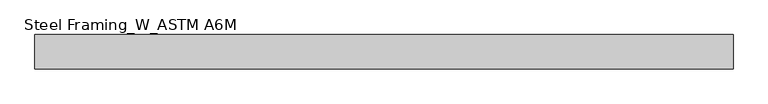
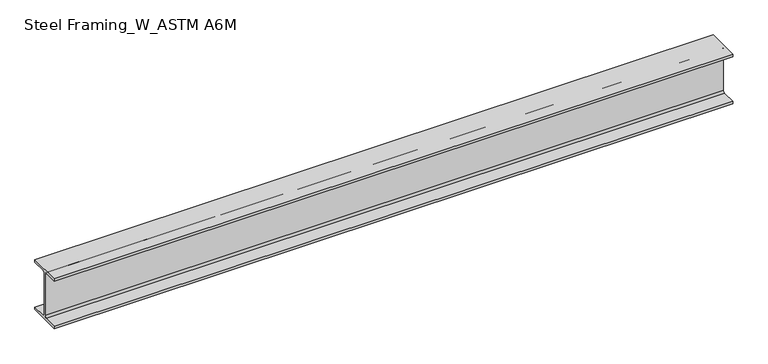
"""IFC4 building model written with IfcOpenShell, lengths in millimetres: beam geometry, Steel Framing_W_ASTM A6M : H_SB_AR_S02_W200x31.3_B6."""

from ifc_helpers import new_model, si_unit, point, frame, frame_2d, origin, place, context, project, spatial, polyline, circle_curve, trimmed, segment, composite_curve, outline, extrude, source, transform, mapped, element, save


def steel_framing_w_astm_a6m_3e5a9afa(model_context):
    return source(origin(), model_context, "Body", "SweptSolid", [
        extrude(outline(composite_curve([segment(polyline([(67.0, -94.8), (67.0, -105.0), (-67.0, -105.0), (-67.0, -94.8), (-10.775, -94.8)]), True, "CONTINUOUS"), segment(trimmed(circle_curve(frame_2d((-10.775, -87.2)), 7.6), [point((-10.775, -94.8))], [point((-3.175, -87.2))], True, "CARTESIAN"), True, "CONTINUOUS"), segment(polyline([(-3.175, -87.2), (-3.175, 87.2)]), True, "CONTINUOUS"), segment(trimmed(circle_curve(frame_2d((-10.775, 87.2)), 7.6), [point((-3.175, 87.2))], [point((-10.775, 94.8))], True, "CARTESIAN"), True, "CONTINUOUS"), segment(polyline([(-10.775, 94.8), (-67.0, 94.8), (-67.0, 105.0), (67.0, 105.0), (67.0, 94.8), (10.775, 94.8)]), True, "CONTINUOUS"), segment(trimmed(circle_curve(frame_2d((10.775, 87.2)), 7.6), [point((10.775, 94.8))], [point((3.175, 87.2))], True, "CARTESIAN"), True, "CONTINUOUS"), segment(polyline([(3.175, 87.2), (3.175, -87.2)]), True, "CONTINUOUS"), segment(trimmed(circle_curve(frame_2d((10.775, -87.2)), 7.6), [point((3.175, -87.2))], [point((10.775, -94.8))], True, "CARTESIAN"), True, "CONTINUOUS"), segment(polyline([(10.775, -94.8), (67.0, -94.8)]), True, "CONTINUOUS")], self_intersect=False)), frame((-1325.5, 0.0, 0.0), z_axis=(1.0, 0.0, 0.0), x_axis=(0.0, 1.0, 0.0)), (0.0, 0.0, 1.0), 2711.8),
    ])


if __name__ == "__main__":
    model = new_model("IFC4")
    model_context = context("Model", 3, world=origin())
    ifc_project = project(units=[si_unit("LENGTHUNIT", "METRE", prefix="MILLI")], contexts=[model_context])
    site = spatial("IfcSite", under=ifc_project)
    building = spatial("IfcBuilding", under=site)
    placement = place(None, origin())
    steel_framing_w_astm_a6m_shape = steel_framing_w_astm_a6m_3e5a9afa(model_context)
    element("IfcBeam", 1, ObjectType="Steel Framing_W_ASTM A6M : H_SB_AR_S02_W200x31.3_B6", at=placement, inside=building, context=model_context, shape_type="MappedRepresentation", body=[
        mapped(steel_framing_w_astm_a6m_shape, transform((0.0, 0.0, 0.0), x_axis=(1.0, 0.0, 0.0), y_axis=(0.0, 1.0, 0.0), z_axis=(0.0, 0.0, 1.0))),
    ])
    save(model, "model.ifc")

# Revit data of these elements
# Type "Steel Framing_W_ASTM A6M : H_SB_AR_S02_W200x31.3_B6"
#   Type Mark = "B6"
#   Section Name Key = "W8x21"
#   Width = 13.4 cm
#   Web Thickness = 0.635 cm
#   Web Fillet = 0.76 cm
#   Warping Constant = 40800.0 cm⁶
#   Torsional Moment of Inertia = 11.70 cm⁴
#   Section Area = 39.7 cm²
#   Plastic Modulus weak axis = 93.2 cm³
#   Plastic Modulus strong axis = 334.0 cm³
#   Perimeter = 0.93 m²/m
#   Nominal Weight = 31.30 kgf/m
#   Moment of Inertia weak axis = 407.00 cm⁴
#   Moment of Inertia strong axis = 3130.00 cm⁴
#   Height = 21.0 cm
#   Flange Thickness = 1.02 cm
#   Elastic Modulus weak axis = 60.8 cm³
#   Elastic Modulus strong axis = 298.0 cm³
#   Centroid Vertical = 10.5 cm
#   Centroid Horizontal = 6.7 cm
#   Length [instance default] = 1500 mm
#   Structural Material [instance default] = Steel, 45-345
#   Bolt Spacing = 0
#   Assembly Code = ""
# Element 1 (IfcBeam, "Steel Framing_W_ASTM A6M : H_SB_AR_S02_W200x31.3_B6")
#   Materials on its faces: "Steel, 45-345"
# Materials
#   "Steel, 45-345": class "Metal", colour RGB 189 187 185, transparency 0, Description = "Steel 345 MPa", Cost = 0
